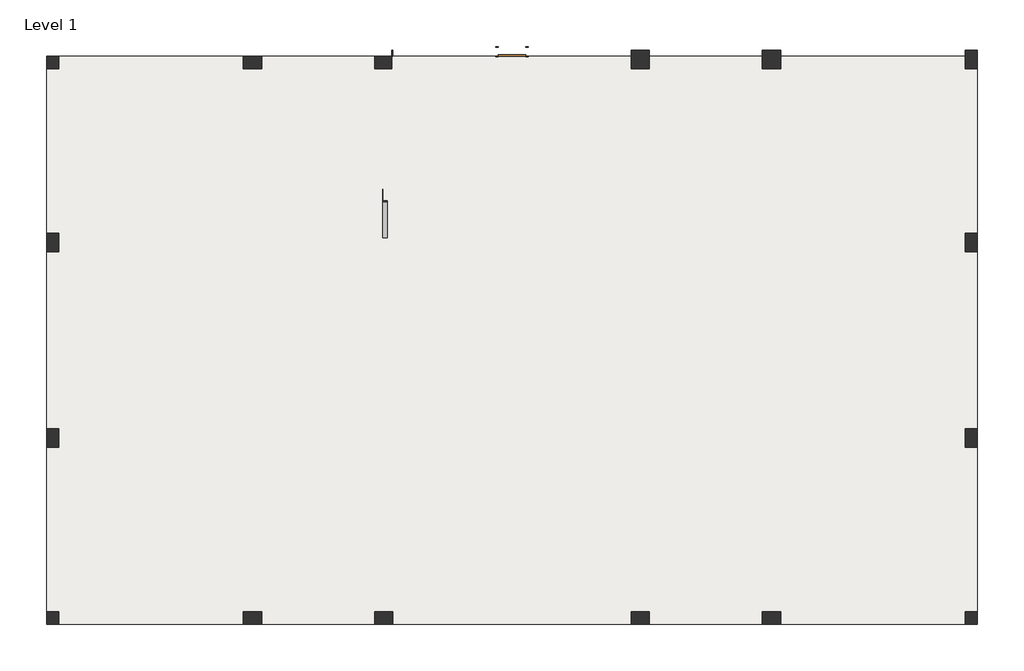
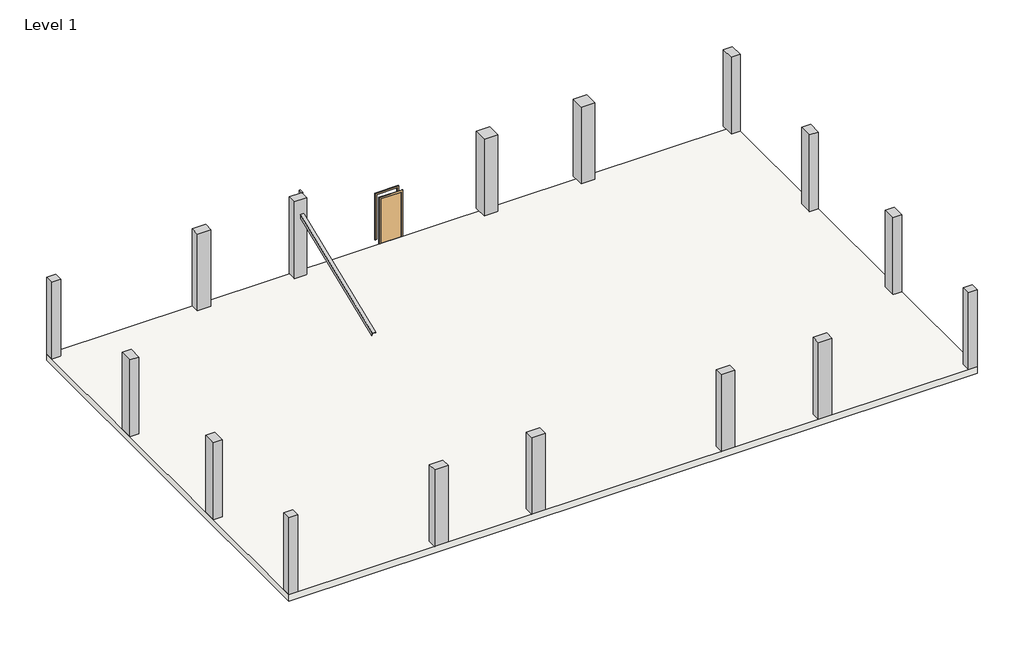
# One storey: 16 columns, 1 door, 1 member, 1 slab.
"""IFC4 building model written with IfcOpenShell, lengths in millimetres."""

import ifcopenshell
import ifcopenshell.guid

model = None  # the IFC model being written
_history = None  # IfcOwnerHistory: only IFC2X3 demands one
_inside = {}  # id of a spatial element -> (the spatial element, [elements in it])
_under = {}  # id of a project, library or spatial element -> (it, [spatial elements below it])
_declared = {}  # id of a project -> (the project, [libraries it declares])
_typed = {}  # id of a type object -> (the type object, [elements of that type])
_made_of = {}  # id of a material, layer set ... -> (it, [elements and type objects made of it])


def new_model(schema):
    """Start an empty IFC model of exactly this schema.

    Asked for "IFC4X3", IfcOpenShell would pick the latest addendum, in which some entities
    have other attributes; the version numbers below select the first issue.
    IFC2X3 requires an IfcOwnerHistory on every rooted entity: one is made here for all.
    """
    global model, _history
    if schema == "IFC4X3":
        model = ifcopenshell.file(schema_version=(4, 3, 0, 0))
    else:
        model = ifcopenshell.file(schema=schema)
    _inside.clear()
    _under.clear()
    _declared.clear()
    _typed.clear()
    _made_of.clear()
    _history = None
    if model.schema == "IFC2X3":
        org = make("IfcOrganization", Name="unknown")
        user = make(
            "IfcPersonAndOrganization",
            ThePerson=make("IfcPerson", FamilyName="unknown"),
            TheOrganization=org,
        )
        app = make(
            "IfcApplication",
            ApplicationDeveloper=org,
            Version="unknown",
            ApplicationFullName="unknown",
            ApplicationIdentifier="unknown",
        )
        _history = make(
            "IfcOwnerHistory",
            OwningUser=user,
            OwningApplication=app,
            ChangeAction="ADDED",
            CreationDate=0,
        )
    return model


def make(cls, **values):
    """One entity of the class cls with the attributes given. An attribute that is None is left unset."""
    return model.create_entity(
        cls, **{name: value for name, value in values.items() if value is not None}
    )


def rooted(cls, **values):
    """An entity with a GlobalId (a new one), such as an element, a storey or a relation."""
    return make(cls, GlobalId=ifcopenshell.guid.new(), OwnerHistory=_history, **values)


def si_unit(unit_type, name, prefix=None):
    """IfcSIUnit, for example si_unit("LENGTHUNIT", "METRE", prefix="MILLI")."""
    return make("IfcSIUnit", UnitType=unit_type, Prefix=prefix, Name=name)


def assignment(units):
    """IfcUnitAssignment: the units of a project."""
    return None if units is None else make("IfcUnitAssignment", Units=units)


def point(xyz):
    """IfcCartesianPoint."""
    return None if xyz is None else make("IfcCartesianPoint", Coordinates=xyz)


def direction(xyz):
    """IfcDirection."""
    return None if xyz is None else make("IfcDirection", DirectionRatios=xyz)


def frame(location, z_axis=None, x_axis=None):
    """IfcAxis2Placement3D, a coordinate frame: its origin and axes. An axis left out is left unset."""
    return make(
        "IfcAxis2Placement3D",
        Location=point(location),
        Axis=direction(z_axis),
        RefDirection=direction(x_axis),
    )


def frame_2d(location, x_axis=None):
    """IfcAxis2Placement2D, a coordinate frame in the plane: its origin and x axis."""
    return make(
        "IfcAxis2Placement2D", Location=point(location), RefDirection=direction(x_axis)
    )


def origin():
    """The frame at (0, 0, 0) with its axes left unset."""
    return frame((0.0, 0.0, 0.0))


def origin_with_axes():
    """The frame at (0, 0, 0) with the z axis (0, 0, 1) and the x axis (1, 0, 0) written out."""
    return frame((0.0, 0.0, 0.0), z_axis=(0.0, 0.0, 1.0), x_axis=(1.0, 0.0, 0.0))


def place(relative_to, where):
    """IfcLocalPlacement: puts the frame where relative to a parent placement (None: the world)."""
    return make(
        "IfcLocalPlacement", PlacementRelTo=relative_to, RelativePlacement=where
    )


def context(
    kind, dimensions, precision=None, world=None, true_north=None, identifier=None
):
    """IfcGeometricRepresentationContext, for example the 3D "Model" context."""
    return make(
        "IfcGeometricRepresentationContext",
        ContextIdentifier=identifier,
        ContextType=kind,
        CoordinateSpaceDimension=dimensions,
        Precision=precision,
        WorldCoordinateSystem=world,
        TrueNorth=true_north,
    )


def project(units=None, contexts=None):
    """IfcProject with its units and contexts."""
    return rooted(
        "IfcProject",
        Name="project",
        RepresentationContexts=contexts,
        UnitsInContext=assignment(units),
    )


def spatial(cls, under=None, at=None, **own):
    """A site, building, storey or space (cls), placed at a placement, below another one or the project."""
    s = rooted(cls, ObjectPlacement=at, **own)
    if under is not None:
        _under.setdefault(under.id(), (under, []))[1].append(s)
    return s


def polyline(points):
    """IfcPolyline through the points."""
    return make("IfcPolyline", Points=[point(p) for p in points])


def circle_curve(where, radius):
    """IfcCircle in the frame where."""
    return make("IfcCircle", Position=where, Radius=radius)


def trimmed(basis, trim1, trim2, sense, master):
    """IfcTrimmedCurve: the piece of a basis curve between two trims."""
    return make(
        "IfcTrimmedCurve",
        BasisCurve=basis,
        Trim1=trim1,
        Trim2=trim2,
        SenseAgreement=sense,
        MasterRepresentation=master,
    )


def segment(curve, same_sense, transition):
    """IfcCompositeCurveSegment."""
    return make(
        "IfcCompositeCurveSegment",
        Transition=transition,
        SameSense=same_sense,
        ParentCurve=curve,
    )


def composite_curve(segments, self_intersect=None):
    """IfcCompositeCurve: segments joined end to end."""
    return make("IfcCompositeCurve", Segments=segments, SelfIntersect=self_intersect)


def outline(outer, holes=None, kind="AREA"):
    """IfcArbitraryClosedProfileDef: a profile drawn as a closed curve; with holes, ...WithVoids."""
    if holes is None:
        return make("IfcArbitraryClosedProfileDef", ProfileType=kind, OuterCurve=outer)
    return make(
        "IfcArbitraryProfileDefWithVoids",
        ProfileType=kind,
        OuterCurve=outer,
        InnerCurves=holes,
    )


def extrude(swept, where, along, depth):
    """IfcExtrudedAreaSolid: the profile swept, set in the frame where, extruded along a direction by depth."""
    return make(
        "IfcExtrudedAreaSolid",
        SweptArea=swept,
        Position=where,
        ExtrudedDirection=direction(along),
        Depth=depth,
    )


def shape(context_of_items, identifier, shape_type, items):
    """IfcShapeRepresentation: the items that make up one representation, for example the "Body"."""
    return make(
        "IfcShapeRepresentation",
        ContextOfItems=context_of_items,
        RepresentationIdentifier=identifier,
        RepresentationType=shape_type,
        Items=items,
    )


def source(mapping_origin, context_of_items, identifier, shape_type, items):
    """IfcRepresentationMap: a shape defined once, which mapped items show again and again."""
    return make(
        "IfcRepresentationMap",
        MappingOrigin=mapping_origin,
        MappedRepresentation=shape(context_of_items, identifier, shape_type, items),
    )


def transform(
    local_origin,
    x_axis=None,
    y_axis=None,
    z_axis=None,
    scale=None,
    scale2=None,
    scale3=None,
    uniform=True,
):
    """IfcCartesianTransformationOperator3D, or its non-uniform kind. x_axis, y_axis, z_axis: its Axis1, 2, 3."""
    if uniform:
        return make(
            "IfcCartesianTransformationOperator3D",
            Axis1=direction(x_axis),
            Axis2=direction(y_axis),
            LocalOrigin=point(local_origin),
            Scale=scale,
            Axis3=direction(z_axis),
        )
    return make(
        "IfcCartesianTransformationOperator3DnonUniform",
        Axis1=direction(x_axis),
        Axis2=direction(y_axis),
        LocalOrigin=point(local_origin),
        Scale=scale,
        Axis3=direction(z_axis),
        Scale2=scale2,
        Scale3=scale3,
    )


def mapped(mapping_source, mapping_target):
    """IfcMappedItem: shows the shape of a source again, moved by a transform."""
    return make(
        "IfcMappedItem", MappingSource=mapping_source, MappingTarget=mapping_target
    )


def made_of(thing, what):
    """Note that an element or type object is made of a material, layer set ...; save() writes the relation."""
    if what is not None:
        _made_of.setdefault(what.id(), (what, []))[1].append(thing)
    return thing


def element(
    cls,
    number,
    at=None,
    inside=None,
    cuts=None,
    type_object=None,
    material=None,
    context=None,
    identifier="Body",
    shape_type=None,
    held_by="IfcProductDefinitionShape",
    body=None,
    shapes=None,
    **own,
):
    """One element of the class cls, such as IfcWall. Its Tag is "e" and its number.

    at: its placement. inside: the storey or other place that contains it. cuts: it is an
    opening in that element (IfcRelVoidsElement). A single representation is given by context,
    identifier, shape_type and body (its items); several are given by shapes. held_by: the class
    of the entity that holds the representations. save() writes the other relations.
    """
    e = rooted(cls, Tag="e%d" % number, ObjectPlacement=at, **own)
    if body is not None:
        shapes = [shape(context, identifier, shape_type, body)]
    if shapes is not None:
        e.Representation = make(held_by, Representations=shapes)
    if inside is not None:
        _inside.setdefault(inside.id(), (inside, []))[1].append(e)
    if cuts is not None:
        rooted(
            "IfcRelVoidsElement", RelatingBuildingElement=cuts, RelatedOpeningElement=e
        )
    if type_object is not None:
        _typed.setdefault(type_object.id(), (type_object, []))[1].append(e)
    return made_of(e, material)


def aggregate(whole, parts):
    """IfcRelAggregates: a whole, such as a stair, and the parts it consists of."""
    return rooted("IfcRelAggregates", RelatingObject=whole, RelatedObjects=parts)


def save(model, path):
    """Write the relations noted so far, then the file.

    IfcRelAggregates (storeys below a building ...), IfcRelContainedInSpatialStructure (elements
    in a storey), IfcRelDefinesByType, IfcRelAssociatesMaterial and IfcRelDeclares: one each for
    every whole, place, type object, material and project.
    """
    for whole, parts in _under.values():
        aggregate(whole, parts)
    for where, things in _inside.values():
        rooted(
            "IfcRelContainedInSpatialStructure",
            RelatedElements=things,
            RelatingStructure=where,
        )
    for kind, things in _typed.values():
        rooted("IfcRelDefinesByType", RelatedObjects=things, RelatingType=kind)
    for what, things in _made_of.values():
        rooted("IfcRelAssociatesMaterial", RelatedObjects=things, RelatingMaterial=what)
    for by, libraries in _declared.values():
        rooted("IfcRelDeclares", RelatingContext=by, RelatedDefinitions=libraries)
    model.write(path)


def door_7b231ec9(model_context):
    return source(origin(), model_context, "Body", "SweptSolid", [
        extrude(outline(polyline([(2209.8, -533.4), (0.0, -533.4), (0.0, -457.2), (2133.6, -457.2), (2133.6, 457.2), (0.0, 457.2), (0.0, 533.4), (2209.8, 533.4), (2209.8, -533.4)])), frame((0.0, 147.6375, 0.0), z_axis=(0.0, 1.0, 0.0), x_axis=(0.0, 0.0, 1.0)), (0.0, 0.0, 1.0), 25.4),
        extrude(outline(polyline([(2209.8, 533.4), (2209.8, -533.4), (0.0, -533.4), (0.0, -457.2), (2133.6, -457.2), (2133.6, 457.2), (0.0, 457.2), (0.0, 533.4), (2209.8, 533.4)])), frame((0.0, -173.0375, 0.0), z_axis=(0.0, 1.0, 0.0), x_axis=(0.0, 0.0, 1.0)), (0.0, 0.0, 1.0), 25.4),
        extrude(outline(polyline([(457.2, 96.8375), (-457.2, 96.8375), (-457.2, 147.6375), (457.2, 147.6375), (457.2, 96.8375)])), origin_with_axes(), (0.0, 0.0, 1.0), 2133.6),
    ])


def l_angle_l6x6x3_8_2b984bf3(model_context):
    return source(origin(), model_context, "Body", "SweptSolid", [
        extrude(outline(composite_curve([segment(polyline([(41.148, 41.148), (41.148, -111.252)]), True, "CONTINUOUS"), segment(trimmed(circle_curve(frame_2d((41.148, -101.727)), 9.525), [point((41.148, -111.252))], [point((31.623, -101.727))], False, "CARTESIAN"), True, "CONTINUOUS"), segment(polyline([(31.623, -101.727), (31.623, 22.098)]), True, "CONTINUOUS"), segment(trimmed(circle_curve(frame_2d((22.098, 22.098)), 9.525), [point((31.623, 22.098))], [point((22.098, 31.623))], True, "CARTESIAN"), True, "CONTINUOUS"), segment(polyline([(22.098, 31.623), (-101.727, 31.623)]), True, "CONTINUOUS"), segment(trimmed(circle_curve(frame_2d((-101.727, 41.148)), 9.525), [point((-101.727, 31.623))], [point((-111.252, 41.148))], False, "CARTESIAN"), True, "CONTINUOUS"), segment(polyline([(-111.252, 41.148), (41.148, 41.148)]), True, "CONTINUOUS")], self_intersect=False)), frame((-3088.1296112, 0.0, 0.0), z_axis=(1.0, 0.0, 0.0), x_axis=(0.0, 1.0, 0.0)), (0.0, 0.0, 1.0), 6142.746295),
    ])


model = new_model("IFC4")

# Units and contexts
model_context = context("Model", 3, world=origin())
ifc_project = project(units=[si_unit("LENGTHUNIT", "METRE", prefix="MILLI")], contexts=[model_context])

# Site, building, storey
site = spatial("IfcSite", under=ifc_project)
building = spatial("IfcBuilding", under=site)
storey = spatial("IfcBuildingStorey", under=building, Name="Level 1", Elevation=0.0)

# Columns
placement = place(None, origin())
element("IfcColumn", 1, ObjectType="Rectangular Column : 24\" x 24\"", at=placement, inside=storey, context=model_context, shape_type="SweptSolid", body=[
    extrude(outline(polyline([(-16253.4122732, 9291.5015304), (-16253.4122732, 8885.1015304), (-16659.8122732, 8885.1015304), (-16659.8122732, 9291.5015304), (-16253.4122732, 9291.5015304)])), origin_with_axes(), (0.0, 0.0, 1.0), 3657.6),
])
element("IfcColumn", 2, ObjectType="Rectangular Column : 24\" x 24\"", at=placement, inside=storey, context=model_context, shape_type="SweptSolid", body=[
    extrude(outline(polyline([(-16253.4122732, 3398.7015304), (-16253.4122732, 2789.1015304), (-16659.8122732, 2789.1015304), (-16659.8122732, 3398.7015304), (-16253.4122732, 3398.7015304)])), origin_with_axes(), (0.0, 0.0, 1.0), 3657.6),
])
element("IfcColumn", 3, ObjectType="Rectangular Column : 24\" x 24\"", at=placement, inside=storey, context=model_context, shape_type="SweptSolid", body=[
    extrude(outline(polyline([(-9497.0122732, 8885.1015304), (-10106.6122732, 8885.1015304), (-10106.6122732, 9291.5015304), (-9497.0122732, 9291.5015304), (-9497.0122732, 8885.1015304)])), origin_with_axes(), (0.0, 0.0, 1.0), 3657.6),
])
element("IfcColumn", 4, ObjectType="Rectangular Column : 24\" x 24\"", at=placement, inside=storey, context=model_context, shape_type="SweptSolid", body=[
    extrude(outline(polyline([(-5174.2497732, 9494.7015304), (-5128.2122732, 9494.7015304), (-5128.2122732, 9301.0265304), (-5174.2497732, 9301.0265304), (-5174.2497732, 9494.7015304)])), origin_with_axes(), (0.0, 0.0, 1.0), 3657.6),
    extrude(outline(polyline([(-5737.8122732, 8885.1015304), (-5737.8122732, 9291.5015304), (-5174.2497732, 9291.5015304), (-5174.2497732, 8885.1015304), (-5737.8122732, 8885.1015304)])), origin_with_axes(), (0.0, 0.0, 1.0), 3657.6),
])
element("IfcColumn", 5, ObjectType="Rectangular Column : 24\" x 24\"", at=placement, inside=storey, context=model_context, shape_type="SweptSolid", body=[
    extrude(outline(polyline([(3406.1877268, 9494.7015304), (3406.1877268, 8885.1015304), (2796.5877268, 8885.1015304), (2796.5877268, 9494.7015304), (3406.1877268, 9494.7015304)])), origin_with_axes(), (0.0, 0.0, 1.0), 3657.6),
])
element("IfcColumn", 6, ObjectType="Rectangular Column : 24\" x 24\"", at=placement, inside=storey, context=model_context, shape_type="SweptSolid", body=[
    extrude(outline(polyline([(7774.9877268, 9494.7015304), (7774.9877268, 8885.1015304), (7165.3877268, 8885.1015304), (7165.3877268, 9494.7015304), (7774.9877268, 9494.7015304)])), origin_with_axes(), (0.0, 0.0, 1.0), 3657.6),
])
element("IfcColumn", 7, ObjectType="Rectangular Column : 24\" x 24\"", at=placement, inside=storey, context=model_context, shape_type="SweptSolid", body=[
    extrude(outline(polyline([(13921.7877268, 8885.1015304), (13921.7877268, 9494.7015304), (14328.1877268, 9494.7015304), (14328.1877268, 8885.1015304), (13921.7877268, 8885.1015304)])), origin_with_axes(), (0.0, 0.0, 1.0), 3657.6),
])
element("IfcColumn", 8, ObjectType="Rectangular Column : 24\" x 24\"", at=placement, inside=storey, context=model_context, shape_type="SweptSolid", body=[
    extrude(outline(polyline([(13921.7877268, 2789.1015304), (13921.7877268, 3398.7015304), (14328.1877268, 3398.7015304), (14328.1877268, 2789.1015304), (13921.7877268, 2789.1015304)])), origin_with_axes(), (0.0, 0.0, 1.0), 3657.6),
])
element("IfcColumn", 9, ObjectType="Rectangular Column : 24\" x 24\"", at=placement, inside=storey, context=model_context, shape_type="SweptSolid", body=[
    extrude(outline(polyline([(13921.7877268, -3713.2984696), (13921.7877268, -3103.6984696), (14328.1877268, -3103.6984696), (14328.1877268, -3713.2984696), (13921.7877268, -3713.2984696)])), origin_with_axes(), (0.0, 0.0, 1.0), 3657.6),
])
element("IfcColumn", 10, ObjectType="Rectangular Column : 24\" x 24\"", at=placement, inside=storey, context=model_context, shape_type="SweptSolid", body=[
    extrude(outline(polyline([(13921.7877268, -9606.0984696), (13921.7877268, -9199.6984696), (14328.1877268, -9199.6984696), (14328.1877268, -9606.0984696), (13921.7877268, -9606.0984696)])), origin_with_axes(), (0.0, 0.0, 1.0), 3657.6),
])
element("IfcColumn", 11, ObjectType="Rectangular Column : 24\" x 24\"", at=placement, inside=storey, context=model_context, shape_type="SweptSolid", body=[
    extrude(outline(polyline([(7165.3877268, -9199.6984696), (7774.9877268, -9199.6984696), (7774.9877268, -9606.0984696), (7165.3877268, -9606.0984696), (7165.3877268, -9199.6984696)])), origin_with_axes(), (0.0, 0.0, 1.0), 3657.6),
])
element("IfcColumn", 12, ObjectType="Rectangular Column : 24\" x 24\"", at=placement, inside=storey, context=model_context, shape_type="SweptSolid", body=[
    extrude(outline(polyline([(2796.5877268, -9199.6984696), (3406.1877268, -9199.6984696), (3406.1877268, -9606.0984696), (2796.5877268, -9606.0984696), (2796.5877268, -9199.6984696)])), origin_with_axes(), (0.0, 0.0, 1.0), 3657.6),
])
element("IfcColumn", 13, ObjectType="Rectangular Column : 24\" x 24\"", at=placement, inside=storey, context=model_context, shape_type="SweptSolid", body=[
    extrude(outline(polyline([(-5737.8122732, -9199.6984696), (-5128.2122732, -9199.6984696), (-5128.2122732, -9606.0984696), (-5737.8122732, -9606.0984696), (-5737.8122732, -9199.6984696)])), origin_with_axes(), (0.0, 0.0, 1.0), 3657.6),
])
element("IfcColumn", 14, ObjectType="Rectangular Column : 24\" x 24\"", at=placement, inside=storey, context=model_context, shape_type="SweptSolid", body=[
    extrude(outline(polyline([(-10106.6122732, -9199.6984696), (-9497.0122732, -9199.6984696), (-9497.0122732, -9606.0984696), (-10106.6122732, -9606.0984696), (-10106.6122732, -9199.6984696)])), origin_with_axes(), (0.0, 0.0, 1.0), 3657.6),
])
element("IfcColumn", 15, ObjectType="Rectangular Column : 24\" x 24\"", at=placement, inside=storey, context=model_context, shape_type="SweptSolid", body=[
    extrude(outline(polyline([(-16659.8122732, -9199.6984696), (-16253.4122732, -9199.6984696), (-16253.4122732, -9606.0984696), (-16659.8122732, -9606.0984696), (-16659.8122732, -9199.6984696)])), origin_with_axes(), (0.0, 0.0, 1.0), 3657.6),
])
element("IfcColumn", 16, ObjectType="Rectangular Column : 24\" x 24\"", at=placement, inside=storey, context=model_context, shape_type="SweptSolid", body=[
    extrude(outline(polyline([(-16253.4122732, -3103.6984696), (-16253.4122732, -3713.2984696), (-16659.8122732, -3713.2984696), (-16659.8122732, -3103.6984696), (-16253.4122732, -3103.6984696)])), origin_with_axes(), (0.0, 0.0, 1.0), 3657.6),
])

# Door
door_shape = door_7b231ec9(model_context)
element("IfcDoor", 17, ObjectType="Single-Flush : 36\" x 84\"", at=placement, inside=storey, context=model_context, shape_type="MappedRepresentation", body=[
    mapped(door_shape, transform((-1165.8122732, 9448.6640304, 0.0), x_axis=(-1.0, 0.0, 0.0), y_axis=(0.0, -1.0, 0.0), z_axis=(0.0, 0.0, 1.0))),
])

# Member
l_angle_l6x6x3_8_shape = l_angle_l6x6x3_8_2b984bf3(model_context)
element("IfcMember", 18, ObjectType="L-Angle : L6X6X3/8", at=placement, inside=storey, context=model_context, shape_type="MappedRepresentation", body=[
    mapped(l_angle_l6x6x3_8_shape, transform((-5433.0122732, 6141.9015304, 1828.8), x_axis=(0.0, 0.9284766908852565, 0.3713906763541112), y_axis=(-1.0000000000000002, 0.0, 0.0), z_axis=(0.0, -0.3713906763541112, 0.9284766908852565))),
])

# Slab
element("IfcSlab", 19, ObjectType="Generic - 12\"", at=placement, inside=storey, context=model_context, shape_type="SweptSolid", body=[
    extrude(outline(polyline([(-16659.8122732, 9291.5015304), (14328.1877268, 9291.5015304), (14328.1877268, -9606.0984696), (-16659.8122732, -9606.0984696), (-16659.8122732, 9291.5015304)])), frame((0.0, 0.0, -304.8), z_axis=(0.0, 0.0, 1.0), x_axis=(1.0, 0.0, 0.0)), (0.0, 0.0, 1.0), 304.8),
])

save(model, "model.ifc")

# Revit data of these elements
# Type "Rectangular Column : 24\" x 24\""
#   Assembly Code = "B1010200"
#   Depth = 2' - 0"
#   Offset Base = 0' - 0"
#   Offset Top = 0' - 0"
#   Width = 2' - 0"
#   Material = none
# Type "Single-Flush : 36\" x 84\""
#   Type Mark = "1"
#   Construction Type Id = "MDOOR"
#   Assembly Code = "C1020"
#   Analytic Construction = "Metal"
#   Thickness = 0' - 2"
#   Heat Transfer Coefficient (U) = 0.651978 BTU/(h·ft²·°F)
#   Height = 7' - 0"
#   Trim Projection Ext = 0' - 1"
#   Trim Projection Int = 0' - 1"
#   Trim Width = 0' - 3"
#   Width = 3' - 0"
#   Define Thermal Properties by = 1
#   Define Thermal Properties by = 1
#   Door Material = Door - Panel
#   Frame Material = Door - Frame
#   Visual Light Transmittance = 0
#   Solar Heat Gain Coefficient = 0
#   Function = (empty or 0)
#   Wall Closure = (empty or 0)
# Type "L-Angle : L6X6X3/8"
#   Assembly Code = "B10"
#   k = 0' - 0 7/8"
#   W = 14.9
#   Length [instance default] = 5' - 0"
#   b = 0' - 6"
#   d = 0' - 6"
#   t = 0' - 0 3/8"
#   x = 0' - 1.62"
#   y = 0' - 1.62"
#   A = 0.0304167 SF
#   Structural Material [instance default] = Steel ASTM A36
# Type "Generic - 12\""
#   Assembly Code = "B1010"
#   Function = 0
#   Layers, outside or top first: 1' - 0" no material (function 1)
# Elements 1, 2, 3, 4, 7, 8, 9, 10, 11, 12, 13, 14, 15, 16 (IfcColumn, "Rectangular Column : 24\" x 24\"")
#   Phase Created = New Construction
#   Materials on its faces: "Default Wall"
# Elements 5, 6 (IfcColumn, "Rectangular Column : 24\" x 24\"")
#   Phase Created = New Construction
# Element 17 (IfcDoor, "Single-Flush : 36\" x 84\"")
#   Phase Created = New Construction
#   Materials on its faces: "Door - Frame", "Door - Panel"
# Element 18 (IfcMember, "L-Angle : L6X6X3/8")
#   Structural Material = Steel ASTM A36
#   Phase Created = New Construction
#   Materials on its faces: "Steel ASTM A36"
# Element 19 (IfcSlab, "Generic - 12\"")
#   built-in parameter 1001955 = 1.5708 (stored number, unit not read)
#   Height Offset From Level = 0' - 0"
#   Phase Created = New Construction
#   Materials on its faces: "Default Floor"
# Materials
#   "Door - Panel": class "Wood", colour RGB 210 159 95, transparency 0, Cost = 0
#   "Door - Frame": class "Miscellaneous", colour RGB 118 70 51, transparency 0, Cost = 0
#   "Steel ASTM A36": class "Metal", colour RGB 199 199 199, transparency 0, Description = "Structural steel, ASTM A36 Grade B, mill finish", Cost = 0
#   "Default Wall": class "Miscellaneous", colour RGB 128 128 128, transparency 0, Cost = 0
#   "Default Floor": class "Miscellaneous", colour RGB 128 128 128, transparency 0, Cost = 0
